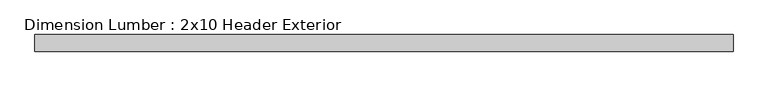
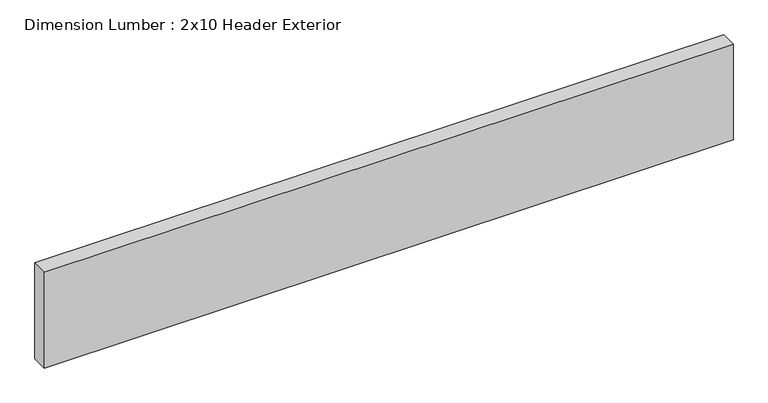
"""IFC4 building model written with IfcOpenShell, lengths in millimetres: beam geometry, Dimension Lumber : 2x10 Header Exterior."""

from ifc_helpers import new_model, si_unit, frame, origin, place, context, project, spatial, polyline, outline, extrude, source, transform, mapped, element, save


def dimension_lumber_2x10_header_exterior_15155622(model_context):
    return source(origin(), model_context, "Body", "SweptSolid", [
        extrude(outline(polyline([(468.709375, 19.05), (468.709375, -19.05), (-1131.490625, -19.05), (-1131.490625, 19.05), (468.709375, 19.05)])), frame((0.0, 0.0, -117.475), z_axis=(0.0, 0.0, 1.0), x_axis=(1.0, 0.0, 0.0)), (0.0, 0.0, 1.0), 234.95),
    ])


if __name__ == "__main__":
    model = new_model("IFC4")
    model_context = context("Model", 3, world=origin())
    ifc_project = project(units=[si_unit("LENGTHUNIT", "METRE", prefix="MILLI")], contexts=[model_context])
    site = spatial("IfcSite", under=ifc_project)
    building = spatial("IfcBuilding", under=site)
    placement = place(None, origin())
    dimension_lumber_2x10_header_exterior_shape = dimension_lumber_2x10_header_exterior_15155622(model_context)
    element("IfcBeam", 1, ObjectType="Dimension Lumber : 2x10 Header Exterior", at=placement, inside=building, context=model_context, shape_type="MappedRepresentation", body=[
        mapped(dimension_lumber_2x10_header_exterior_shape, transform((0.0, 0.0, 0.0), x_axis=(1.0, 0.0, 0.0), y_axis=(0.0, 1.0, 0.0), z_axis=(0.0, 0.0, 1.0))),
    ])
    save(model, "model.ifc")

# Revit data of these elements
# Type "Dimension Lumber : 2x10 Header Exterior"
#   Assembly Code = "B10"
#   A = 0.0963889 SF
#   Length [instance default] = 5' - 0"
#   b = 0' - 1 1/2"
#   d = 0' - 9 1/4"
#   Structural Material [instance default] = Softwood, Lumber
# Element 1 (IfcBeam, "Dimension Lumber : 2x10 Header Exterior")
#   Structural Material = Douglas Fir #2
#   Materials on its faces: "Douglas Fir #2"
# Materials
#   "Softwood, Lumber": class "Wood", colour RGB 223 192 134, transparency 0, Description = "Pinus Echinata", Cost = 0
#   "Douglas Fir #2": class "Wood", colour RGB 223 192 134, transparency 0, Description = "Pinus Echinata", Cost = 0
